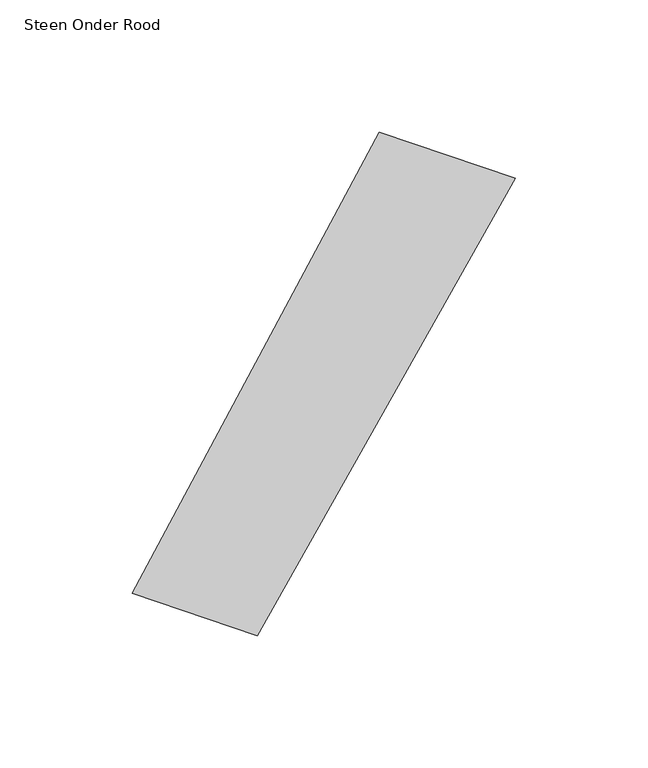
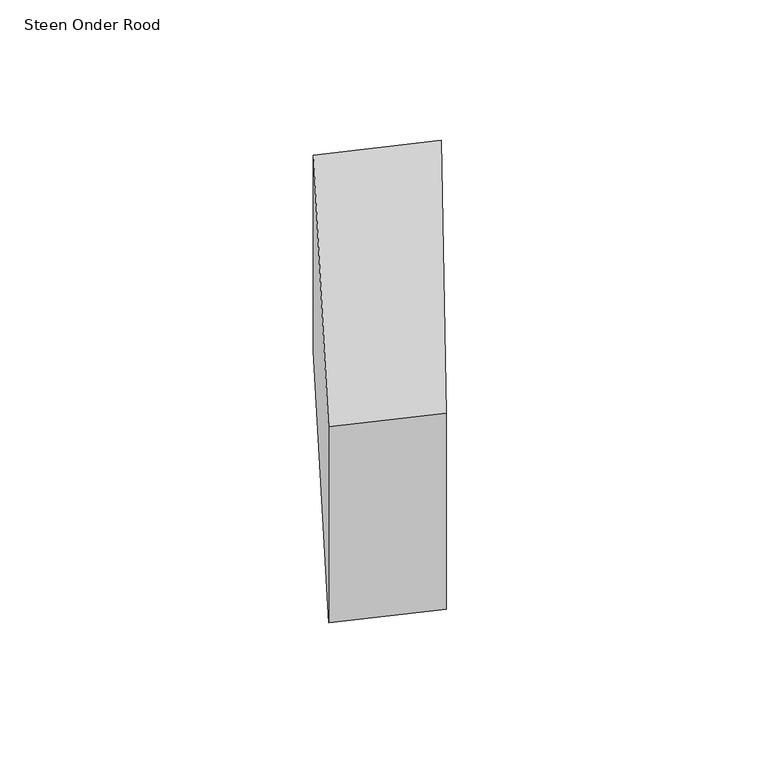
"""IFC4 building model written with IfcOpenShell, lengths in millimetres: proxy geometry, 00_GMA_steen_versie_4 : Steen Onder Rood."""

from ifc_helpers import new_model, si_unit, origin, origin_with_axes, place, context, project, spatial, polyline, outline, extrude, source, transform, mapped, element, save


def steen_onder_rood_8bb4a415(model_context):
    return source(origin(), model_context, "Body", "SweptSolid", [
        extrude(outline(polyline([(148.3328985, 154.4980521), (50.8463023, -18.4545027), (3.4890538, -2.4142092), (96.8614436, 171.9150537), (148.3328985, 154.4980521)])), origin_with_axes(), (0.0, 0.0, 1.0), 100.0),
    ])


if __name__ == "__main__":
    model = new_model("IFC4")
    model_context = context("Model", 3, world=origin())
    ifc_project = project(units=[si_unit("LENGTHUNIT", "METRE", prefix="MILLI")], contexts=[model_context])
    site = spatial("IfcSite", under=ifc_project)
    building = spatial("IfcBuilding", under=site)
    placement = place(None, origin())
    steen_onder_rood_shape = steen_onder_rood_8bb4a415(model_context)
    element("IfcBuildingElementProxy", 1, Name="00_GMA_steen_versie_4 : Steen Onder Rood", ObjectType="00_GMA_steen_versie_4 : Steen Onder Rood", at=placement, inside=building, context=model_context, shape_type="MappedRepresentation", body=[
        mapped(steen_onder_rood_shape, transform((0.0, 0.0, 0.0), x_axis=(1.0, 0.0, 0.0), y_axis=(0.0, 1.0, 0.0), z_axis=(0.0, 0.0, 1.0))),
    ])
    save(model, "model.ifc")

# Revit data of these elements
# Type "00_GMA_steen_versie_4 : Steen Onder Rood"
#   StootVoegHalfBoven [instance default] = 5 mm
#   StootVoegHalf [instance default] = 5 mm
#   StootVoegBreedteOnder = 10 mm
#   StootVoegBreedteBoven = 10 mm
#   Steendikte = 100 mm
#   LintVoegOnderHalf = 0 mm
#   LintVoegOnder = 0 mm
#   LintVoegBovenHalf = 5 mm
#   LintVoegBoven = 10 mm
#   materiaal = 21_steen_rood
#   MateriaalVoeg = none
#   Default Elevation = 0
# Element 1 (IfcBuildingElementProxy, "00_GMA_steen_versie_4 : Steen Onder Rood")
#   Materials on its faces: "21_steen_rood"
# Materials
#   "21_steen_rood": class "Unassigned", colour RGB 213 111 43, transparency 0, Cost = 0
